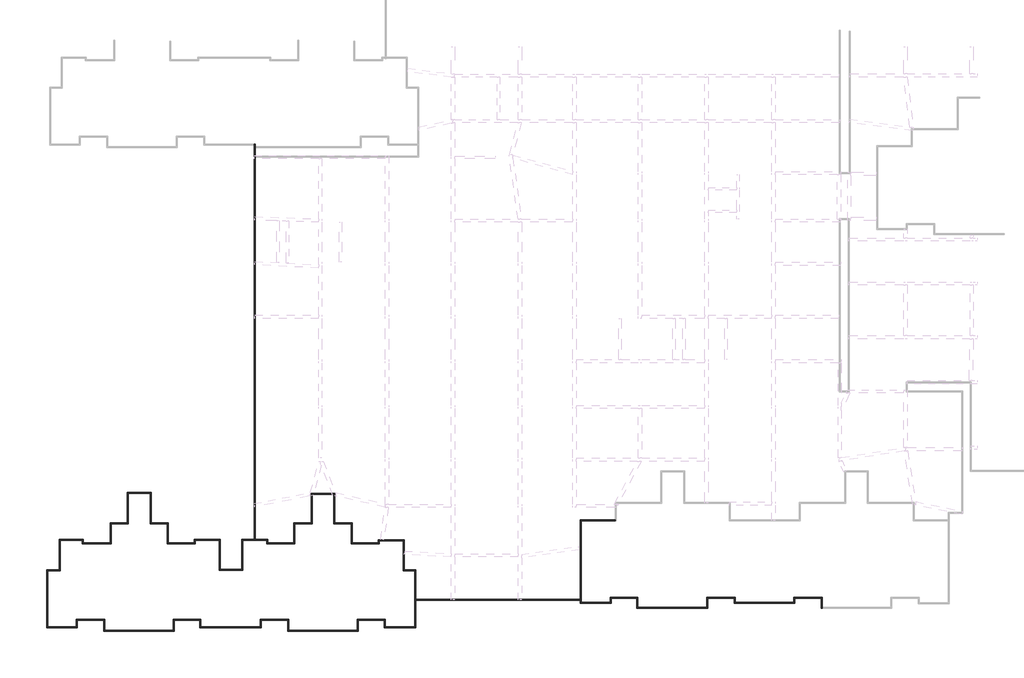
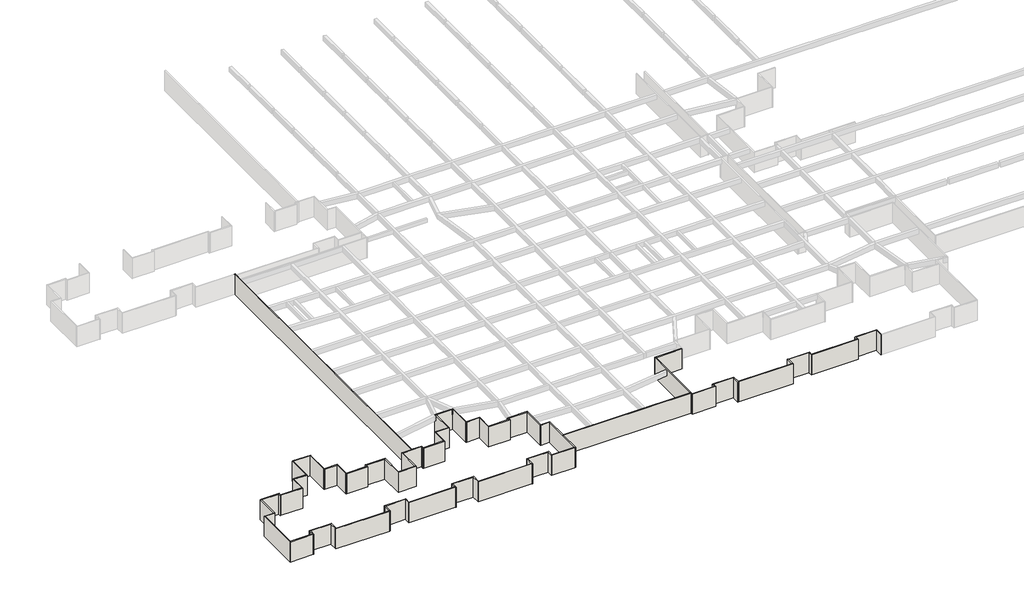
# One storey, part 1 of 16: 68 walls.
# Revit data of these elements (continued)
# Area, not placed, upper offset 0 mm, lower offset 0 mm
#   Number = "24"
#   Name = "fire_compart"
# Area, not placed, upper offset 0 mm, lower offset 0 mm
#   Number = "103"
#   Name = "main_building"
# Area, not placed, upper offset 0 mm, lower offset 0 mm
#   Number = "58"
#   Name = "fire_compart"
# Area, not placed, upper offset 0 mm, lower offset 0 mm
#   Number = "98"
#   Name = "fire_compart"
# Area, not placed, upper offset 0 mm, lower offset 0 mm
#   Number = "99"
#   Name = "main_building"
# Area, not placed, upper offset 0 mm, lower offset 0 mm
#   Number = "123"
#   Name = "main_building"
# Area, not placed, upper offset 0 mm, lower offset 0 mm
#   Number = "59"
#   Name = "fire_compart"
# Room, not placed, phase "新构造", upper offset 0 mm, lower offset 0 mm
#   Number = "1"
#   Name = "客餐厅"
# Room, not placed, phase "新构造", upper offset 0 mm, lower offset 0 mm
#   Number = "2"
#   Name = "阳台"
# Room, not placed, phase "新构造", upper offset 0 mm, lower offset 0 mm
#   Number = "3"
#   Name = "次卧"
# Room, not placed, phase "新构造", upper offset 0 mm, lower offset 0 mm
#   Number = "4"
#   Name = "厨房"
# Area, not placed, upper offset 0 mm, lower offset 0 mm
#   Number = "108"
#   Name = "main_building"
# Room, not placed, phase "新构造", upper offset 0 mm, lower offset 0 mm
#   Number = "5"
#   Name = "卫生间"
# Room, not placed, phase "新构造", upper offset 0 mm, lower offset 0 mm
#   Number = "6"
#   Name = "次卧"
# Room, not placed, phase "新构造", upper offset 0 mm, lower offset 0 mm
#   Number = "7"
#   Name = "主卧"
# Area, not placed, upper offset 0 mm, lower offset 0 mm
#   Number = "60"
#   Name = "fire_compart"
# Area, not placed, upper offset 0 mm, lower offset 0 mm
#   Number = "23"
#   Name = "main_building"
# Area, not placed, upper offset 0 mm, lower offset 0 mm
#   Number = "124"
#   Name = "fire_compart"
# Area, not placed, upper offset 0 mm, lower offset 0 mm
#   Number = "36"
#   Name = "main_building"
# Area, not placed, upper offset 0 mm, lower offset 0 mm
#   Number = "37"
#   Name = "main_building"
# Area, not placed, upper offset 0 mm, lower offset 0 mm
#   Number = "38"
#   Name = "main_building"
# Area, not placed, upper offset 0 mm, lower offset 0 mm
#   Number = "39"
#   Name = "main_building"
# Area, not placed, upper offset 0 mm, lower offset 0 mm
#   Number = "40"
#   Name = "main_building"
# Area, not placed, upper offset 0 mm, lower offset 0 mm
#   Number = "64"
#   Name = "fire_compart"
# Area, not placed, upper offset 0 mm, lower offset 0 mm
#   Number = "61"
#   Name = "fire_compart"
# Area, not placed, upper offset 0 mm, lower offset 0 mm
#   Number = "65"
#   Name = "main_building"
# Area, not placed, upper offset 0 mm, lower offset 0 mm
#   Number = "104"
#   Name = "main_building"
# Area, not placed, upper offset 0 mm, lower offset 0 mm
#   Number = "62"
#   Name = "fire_compart"
# Area at (368764.448, -121371.747) mm, upper offset 0 mm, lower offset 0 mm
#   Number = "163"
#   Name = "main_building"
# Area, not placed, upper offset 0 mm, lower offset 0 mm
#   Number = "125"
#   Name = "fire_compart"
# Area at (211824.528, -122416.854) mm, upper offset 0 mm, lower offset 0 mm
#   Number = "161"
#   Name = "main_building"
# Area, not placed, upper offset 0 mm, lower offset 0 mm
#   Number = "63"
#   Name = "fire_compart"
# Area, not placed, upper offset 0 mm, lower offset 0 mm
#   Number = "66"
#   Name = "main_building"
# Area, not placed, upper offset 0 mm, lower offset 0 mm
#   Number = "126"
#   Name = "fire_compart"
# Area at (352740.132, -178946.021) mm, upper offset 0 mm, lower offset 0 mm
#   Number = "166"
#   Name = "main_building"
# Area, not placed, upper offset 0 mm, lower offset 0 mm
#   Number = "83"
#   Name = "fire_compart"
# Area, not placed, upper offset 0 mm, lower offset 0 mm
#   Number = "84"
#   Name = "main_building"
# Area, not placed, upper offset 0 mm, lower offset 0 mm
#   Number = "150"
#   Name = "main_building"
# Area, not placed, upper offset 0 mm, lower offset 0 mm
#   Number = "127"
#   Name = "fire_compart"
# Area, not placed, upper offset 0 mm, lower offset 0 mm
#   Number = "7"
#   Name = "fire_compart_5"
# Area, not placed, upper offset 0 mm, lower offset 0 mm
#   Number = "128"
#   Name = "fire_compart"
# Area, not placed, upper offset 0 mm, lower offset 0 mm
#   Number = "129"
#   Name = "fire_compart"
# Area, not placed, upper offset 0 mm, lower offset 0 mm
#   Number = "151"
#   Name = "main_building"
# Area, not placed, upper offset 0 mm, lower offset 0 mm
#   Number = "130"
#   Name = "fire_compart"
# Area, not placed, upper offset 0 mm, lower offset 0 mm
#   Number = "109"
#   Name = "main_building"
# Area, not placed, upper offset 0 mm, lower offset 0 mm
#   Number = "67"
#   Name = "fire_compart"
# Area, not placed, upper offset 0 mm, lower offset 0 mm
#   Number = "112"
#   Name = "main_building"
# Area, not placed, upper offset 0 mm, lower offset 0 mm
#   Number = "131"
#   Name = "fire_compart"
# Area, not placed, upper offset 0 mm, lower offset 0 mm
#   Number = "68"
#   Name = "fire_compart"
# Area at (204352.281, -210158.202) mm, upper offset 0 mm, lower offset 0 mm
#   Number = "171"
#   Name = "fire_compart"
# Area, not placed, upper offset 0 mm, lower offset 0 mm
#   Number = "152"
#   Name = "main_building"
# Area, not placed, upper offset 0 mm, lower offset 0 mm
#   Number = "132"
#   Name = "fire_compart"
# Area, not placed, upper offset 0 mm, lower offset 0 mm
#   Number = "1"
#   Name = "面积"
# Area, not placed, upper offset 0 mm, lower offset 0 mm
#   Number = "2"
#   Name = "防火区域1"
# Area at (226846.528, -141041.133) mm, upper offset 0 mm, lower offset 0 mm
#   Number = "172"
#   Name = "fire_compart"
# Area, not placed, upper offset 0 mm, lower offset 0 mm
#   Number = "133"
#   Name = "fire_compart"
# Area, not placed, upper offset 0 mm, lower offset 0 mm
#   Number = "144"
#   Name = "fire_compart"
# Area at (280323.777, -180429.015) mm, upper offset 0 mm, lower offset 0 mm
#   Number = "167"
#   Name = "main_building"
# Area, not placed, upper offset 0 mm, lower offset 0 mm
#   Number = "134"
#   Name = "fire_compart"
# Area at (290707.732, -158085.074) mm, upper offset 0 mm, lower offset 0 mm
#   Number = "173"
#   Name = "fire_compart"
# Area, not placed, upper offset 0 mm, lower offset 0 mm
#   Number = "25"
#   Name = "fire_compart"
# Area, not placed, upper offset 0 mm, lower offset 0 mm
#   Number = "26"
#   Name = "fire_compart"
# Area, not placed, upper offset 0 mm, lower offset 0 mm
#   Number = "27"
#   Name = "fire_compart"
# Area, not placed, upper offset 0 mm, lower offset 0 mm
#   Number = "69"
#   Name = "fire_compart"
# Area, not placed, upper offset 0 mm, lower offset 0 mm
#   Number = "105"
#   Name = "main_building"
# Area, not placed, upper offset 0 mm, lower offset 0 mm
#   Number = "113"
#   Name = "main_building"
# Area, not placed, upper offset 0 mm, lower offset 0 mm
#   Number = "153"
#   Name = "main_building"
# Area, not placed, upper offset 0 mm, lower offset 0 mm
#   Number = "135"
#   Name = "fire_compart"
# Area at (277721.72, -122129.455) mm, upper offset 0 mm, lower offset 0 mm
#   Number = "162"
#   Name = "main_building"
# Area, not placed, upper offset 0 mm, lower offset 0 mm
#   Number = "85"
#   Name = "fire_compart"
# Area, not placed, upper offset 0 mm, lower offset 0 mm
#   Number = "86"
#   Name = "main_building"
# Area, not placed, upper offset 0 mm, lower offset 0 mm
#   Number = "87"
#   Name = "main_building"
# Area at (297761.222, -195328.492) mm, upper offset 0 mm, lower offset 0 mm
#   Number = "174"
#   Name = "fire_compart"
# Area, not placed, upper offset 0 mm, lower offset 0 mm
#   Number = "136"
#   Name = "fire_compart"
# Room, not placed, phase "新构造", upper offset 0 mm, lower offset 0 mm
#   Number = "8"
#   Name = "客餐厅"
# Area, not placed, upper offset 0 mm, lower offset 0 mm
#   Number = "70"
#   Name = "main_building"
# Area, not placed, upper offset 0 mm, lower offset 0 mm
#   Number = "156"
#   Name = "fire_compart"
# Area at (362915.449, -140387.476) mm, upper offset 0 mm, lower offset 0 mm
#   Number = "175"
#   Name = "fire_compart"
# Area, not placed, upper offset 0 mm, lower offset 0 mm
#   Number = "154"
#   Name = "main_building"
# Area at (243225.401, -224393.687) mm, upper offset 0 mm, lower offset 0 mm
#   Number = "168"
#   Name = "main_building"
# Area at (433375.172, -140755.294) mm, upper offset 0 mm, lower offset 0 mm
#   Number = "176"
#   Name = "fire_compart"
# Area, not placed, upper offset 0 mm, lower offset 0 mm
#   Number = "114"
#   Name = "main_building"
# Area, not placed, upper offset 0 mm, lower offset 0 mm
#   Number = "8"
#   Name = "fire_compart_6"
# Area, not placed, upper offset 0 mm, lower offset 0 mm
#   Number = "137"
#   Name = "fire_compart"
# Area, not placed, upper offset 0 mm, lower offset 0 mm
#   Number = "138"
#   Name = "fire_compart"
# Area at (436976.851, -126262.148) mm, upper offset 0 mm, lower offset 0 mm
#   Number = "164"
#   Name = "main_building"
# Area, not placed, upper offset 0 mm, lower offset 0 mm
#   Number = "3"
#   Name = "fire_compart_1"
# Area, not placed, upper offset 0 mm, lower offset 0 mm
#   Number = "139"
#   Name = "fire_compart"
# Area, not placed, upper offset 0 mm, lower offset 0 mm
#   Number = "71"
#   Name = "fire_compart"
# Room, not placed, phase "新构造", upper offset 0 mm, lower offset 0 mm
#   Number = "11"
#   Name = "房间"
# Area, not placed, upper offset 0 mm, lower offset 0 mm
#   Number = "140"
#   Name = "fire_compart"
# Area, not placed, upper offset 0 mm, lower offset 0 mm
#   Number = "155"
#   Name = "main_building"
# Area, not placed, upper offset 0 mm, lower offset 0 mm
#   Number = "106"
#   Name = "main_building"
# Room, not placed, phase "新构造", upper offset 0 mm, lower offset 0 mm
#   Number = "12"
#   Name = "房间"
# Area, not placed, upper offset 0 mm, lower offset 0 mm
#   Number = "110"
#   Name = "main_building"
# Area, not placed, upper offset 0 mm, lower offset 0 mm
#   Number = "115"
#   Name = "main_building"
# Area, not placed, upper offset 0 mm, lower offset 0 mm
#   Number = "141"
#   Name = "fire_compart"
# Area, not placed, upper offset 0 mm, lower offset 0 mm
#   Number = "100"
#   Name = "main_building"
# Room, not placed, phase "新构造", upper offset 0 mm, lower offset 0 mm
#   Number = "13"
#   Name = "房间"
# Room, not placed, phase "新构造", upper offset 0 mm, lower offset 0 mm
#   Number = "14"
#   Name = "房间"
# Area, not placed, upper offset 0 mm, lower offset 0 mm
#   Number = "72"
#   Name = "main_building"
# Room, not placed, phase "新构造", upper offset 0 mm, lower offset 0 mm
#   Number = "15"
#   Name = "房间"
# Area, not placed, upper offset 0 mm, lower offset 0 mm
#   Number = "88"
#   Name = "fire_compart"
# Room, not placed, phase "新构造", upper offset 0 mm, lower offset 0 mm
#   Number = "16"
#   Name = "房间"
# Area, not placed, upper offset 0 mm, lower offset 0 mm
#   Number = "28"
#   Name = "面积"
# Area, not placed, upper offset 0 mm, lower offset 0 mm
#   Number = "73"
#   Name = "fire_compart"
# Area, not placed, upper offset 0 mm, lower offset 0 mm
#   Number = "116"
#   Name = "main_building"
# Area at (182783.854, -229295.599) mm, upper offset 0 mm, lower offset 0 mm
#   Number = "169"
#   Name = "main_building"
# Area, not placed, upper offset 0 mm, lower offset 0 mm
#   Number = "101"
#   Name = "main_building"
# Room, not placed, phase "新构造", upper offset 0 mm, lower offset 0 mm
#   Number = "17"
#   Name = "房间"
# Area, not placed, upper offset 0 mm, lower offset 0 mm
#   Number = "30"
#   Name = "main_building"
# Area, not placed, upper offset 0 mm, lower offset 0 mm
#   Number = "143"
#   Name = "fire_compart"
# Area, not placed, upper offset 0 mm, lower offset 0 mm
#   Number = "89"
#   Name = "main_building"
# Area, not placed, upper offset 0 mm, lower offset 0 mm
#   Number = "75"
#   Name = "main_building"
# Area, not placed, upper offset 0 mm, lower offset 0 mm
#   Number = "111"
#   Name = "main_building"
# Area, not placed, upper offset 0 mm, lower offset 0 mm
#   Number = "90"
#   Name = "fire_compart"
# Area, not placed, upper offset 0 mm, lower offset 0 mm
#   Number = "76"
#   Name = "main_building"
# Area, not placed, upper offset 0 mm, lower offset 0 mm
#   Number = "145"
#   Name = "fire_compart"
# Area, not placed, upper offset 0 mm, lower offset 0 mm
#   Number = "146"
#   Name = "fire_compart"
# Area, not placed, upper offset 0 mm, lower offset 0 mm
#   Number = "147"
#   Name = "fire_compart"
# Area, not placed, upper offset 0 mm, lower offset 0 mm
#   Number = "117"
#   Name = "main_building"
# Area, not placed, upper offset 0 mm, lower offset 0 mm
#   Number = "4"
#   Name = "fire_compart_2"
# Area, not placed, upper offset 0 mm, lower offset 0 mm
#   Number = "77"
#   Name = "main_building"
# Area, not placed, upper offset 0 mm, lower offset 0 mm
#   Number = "159"
#   Name = "fire_compart"
# Area, not placed, upper offset 0 mm, lower offset 0 mm
#   Number = "78"
#   Name = "main_building"
# Area, not placed, upper offset 0 mm, lower offset 0 mm
#   Number = "79"
#   Name = "main_building"
# Area, not placed, upper offset 0 mm, lower offset 0 mm
#   Number = "29"
#   Name = "main_building"
